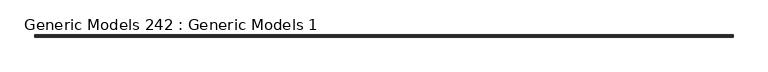
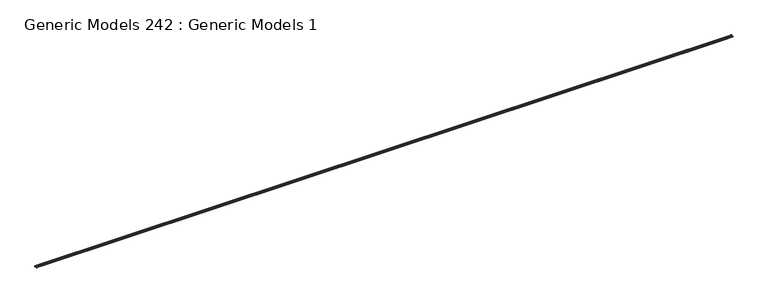
"""IFC4 building model written with IfcOpenShell, lengths in millimetres: proxy geometry, Generic Models 242 : Generic Models 1."""

from ifc_helpers import new_model, si_unit, origin, place, context, project, spatial, faceted_brep, source, transform, mapped, element, save


def generic_models_242_generic_models_1_e672850e(model_context):
    return source(origin(), model_context, "Body", "Brep", [
        faceted_brep([(-5248.1628079, -20076.4173745, 126772.8249329), (-5248.1628079, -20076.4173745, 126775.0347329), (-5248.1628079, -20077.2762154, 126775.0347329), (-5248.1628079, -20077.2762154, 126795.3493116), (-5248.1628079, -20076.0062154, 126795.3493116), (-5248.1628079, -20076.0062154, 126776.3047329), (-5248.1628079, -20075.1473745, 126776.3047329), (-5248.1628079, -20075.1473745, 126771.5549329), (-5248.1628079, -20097.3723745, 126771.5549329), (-5248.1628079, -20097.3723745, 126782.9849329), (-5248.1628079, -20110.0723745, 126782.9849329), (-5248.1628079, -20110.0723745, 126771.5549329), (-5248.1628079, -20133.7855584, 126771.5549329), (-5248.1628079, -20133.7855584, 126772.8249329), (-5248.1628079, -20111.3423745, 126772.8249329), (-5248.1628079, -20111.3423745, 126784.2549329), (-5248.1628079, -20096.1023745, 126784.2549329), (-5248.1628079, -20096.1023745, 126772.8249329), (13801.8371921, -20076.4173745, 126772.8249329), (13801.8371921, -20096.1023745, 126772.8249329), (13801.8371921, -20096.1023745, 126784.2549329), (13801.8371921, -20111.3423745, 126784.2549329), (13801.8371921, -20111.3423745, 126772.8249329), (13801.8371921, -20133.7855584, 126772.8249329), (13801.8371921, -20133.7855584, 126771.5549329), (13801.8371921, -20110.0723745, 126771.5549329), (13801.8371921, -20110.0723745, 126782.9849329), (13801.8371921, -20097.3723745, 126782.9849329), (13801.8371921, -20097.3723745, 126771.5549329), (13801.8371921, -20075.1473745, 126771.5549329), (13801.8371921, -20075.1473745, 126776.3047329), (13801.8371921, -20076.0062154, 126776.3047329), (13801.8371921, -20076.0062154, 126795.3493116), (13801.8371921, -20077.2762154, 126795.3493116), (13801.8371921, -20077.2762154, 126775.0347329), (13801.8371921, -20076.4173745, 126775.0347329), (13576.4121921, -20133.7855584, 126771.5549329), (-5067.1878079, -20133.7855584, 126771.5549329), (13576.4121921, -20133.7855584, 126772.8249329), (-5067.1878079, -20133.7855584, 126772.8249329), (13576.4121921, -20111.3423745, 126772.8249329), (-5067.1878079, -20111.3423745, 126772.8249329)], [[[0, 1, 2, 3, 4, 5, 6, 7, 8, 9, 10, 11, 12, 13, 14, 15, 16, 17]], [[18, 19, 20, 21, 22, 23, 24, 25, 26, 27, 28, 29, 30, 31, 32, 33, 34, 35]], [[1, 0, 18, 35]], [[2, 1, 35, 34]], [[3, 2, 34, 33]], [[4, 3, 33, 32]], [[5, 4, 32, 31]], [[6, 5, 31, 30]], [[7, 6, 30, 29]], [[8, 7, 29, 28]], [[9, 8, 28, 27]], [[10, 9, 27, 26]], [[11, 10, 26, 25]], [[12, 11, 25, 24, 36, 37]], [[13, 12, 37, 36, 24, 23, 38, 39]], [[14, 13, 39, 38, 23, 22, 40, 41]], [[15, 14, 41, 40, 22, 21]], [[16, 15, 21, 20]], [[17, 16, 20, 19]], [[0, 17, 19, 18]]]),
    ])


if __name__ == "__main__":
    model = new_model("IFC4")
    model_context = context("Model", 3, world=origin())
    ifc_project = project(units=[si_unit("LENGTHUNIT", "METRE", prefix="MILLI")], contexts=[model_context])
    site = spatial("IfcSite", under=ifc_project)
    building = spatial("IfcBuilding", under=site)
    placement = place(None, origin())
    generic_models_242_generic_models_1_shape = generic_models_242_generic_models_1_e672850e(model_context)
    element("IfcBuildingElementProxy", 1, Name="Generic Models 242 : Generic Models 1", ObjectType="Generic Models 242 : Generic Models 1", at=placement, inside=building, context=model_context, shape_type="MappedRepresentation", body=[
        mapped(generic_models_242_generic_models_1_shape, transform((0.0, 0.0, 0.0), x_axis=(1.0, 0.0, 0.0), y_axis=(0.0, 1.0, 0.0), z_axis=(0.0, 0.0, 1.0))),
    ])
    save(model, "model.ifc")

# Revit data of these elements
# Element 1 (IfcBuildingElementProxy, "Generic Models 242 : Generic Models 1")
#   Materials on its faces: "_16 GA. COPPER SOFFIT DRIP SCREED"
# Materials
#   "_16 GA. COPPER SOFFIT DRIP SCREED": class "Generic", colour RGB 253 192 103, transparency 0, Cost = 0
